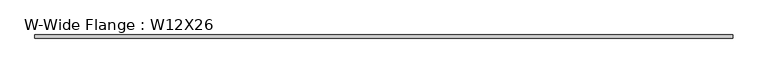
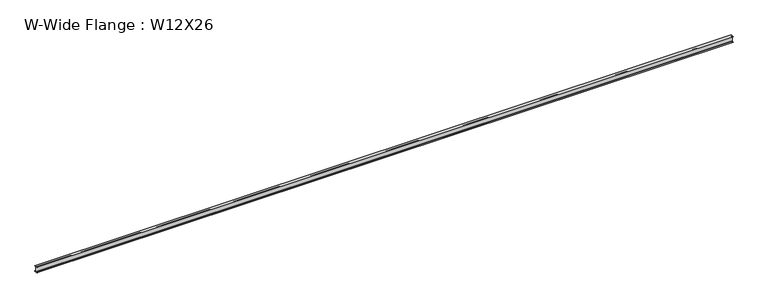
"""IFC4 building model written with IfcOpenShell, lengths in millimetres: beam geometry, W-Wide Flange : W12X26."""

from ifc_helpers import new_model, si_unit, point, frame, frame_2d, origin, place, context, project, spatial, polyline, circle_curve, trimmed, segment, composite_curve, outline, extrude, source, transform, mapped, element, save


def w_wide_flange_w12x26_694e4f9e(model_context):
    return source(origin(), model_context, "Body", "SweptSolid", [
        extrude(outline(composite_curve([segment(polyline([(82.4011719, -145.5539063), (82.4011719, -155.178125), (-82.4011719, -155.178125), (-82.4011719, -145.5539063), (-20.2902344, -145.5539063)]), True, "CONTINUOUS"), segment(trimmed(circle_curve(frame_2d((-20.2902344, -128.190625)), 17.3632812), [point((-20.2902344, -145.5539063))], [point((-2.9269531, -128.190625))], True, "CARTESIAN"), True, "CONTINUOUS"), segment(polyline([(-2.9269531, -128.190625), (-2.9269531, 128.190625)]), True, "CONTINUOUS"), segment(trimmed(circle_curve(frame_2d((-20.2902344, 128.190625)), 17.3632812), [point((-2.9269531, 128.190625))], [point((-20.2902344, 145.5539062))], True, "CARTESIAN"), True, "CONTINUOUS"), segment(polyline([(-20.2902344, 145.5539062), (-82.4011719, 145.5539062), (-82.4011719, 155.178125), (82.4011719, 155.178125), (82.4011719, 145.5539062), (20.2902344, 145.5539062)]), True, "CONTINUOUS"), segment(trimmed(circle_curve(frame_2d((20.2902344, 128.190625)), 17.3632812), [point((20.2902344, 145.5539062))], [point((2.9269531, 128.190625))], True, "CARTESIAN"), True, "CONTINUOUS"), segment(polyline([(2.9269531, 128.190625), (2.9269531, -128.190625)]), True, "CONTINUOUS"), segment(trimmed(circle_curve(frame_2d((20.2902344, -128.190625)), 17.3632812), [point((2.9269531, -128.190625))], [point((20.2902344, -145.5539063))], True, "CARTESIAN"), True, "CONTINUOUS"), segment(polyline([(20.2902344, -145.5539063), (82.4011719, -145.5539063)]), True, "CONTINUOUS")], self_intersect=False)), frame((-18165.7496628, 0.0, 0.0), z_axis=(1.0, 0.0, 0.0), x_axis=(0.0, 1.0, 0.0)), (0.0, 0.0, 1.0), 36331.4993256),
    ])


if __name__ == "__main__":
    model = new_model("IFC4")
    model_context = context("Model", 3, world=origin())
    ifc_project = project(units=[si_unit("LENGTHUNIT", "METRE", prefix="MILLI")], contexts=[model_context])
    site = spatial("IfcSite", under=ifc_project)
    building = spatial("IfcBuilding", under=site)
    placement = place(None, origin())
    w_wide_flange_w12x26_shape = w_wide_flange_w12x26_694e4f9e(model_context)
    element("IfcBeam", 1, ObjectType="W-Wide Flange : W12X26", at=placement, inside=building, context=model_context, shape_type="MappedRepresentation", body=[
        mapped(w_wide_flange_w12x26_shape, transform((0.0, 0.0, 0.0), x_axis=(1.0, 0.0, 0.0), y_axis=(0.0, 1.0, 0.0), z_axis=(0.0, 0.0, 1.0))),
    ])
    save(model, "model.ifc")

# Revit data of these elements
# Type "W-Wide Flange : W12X26"
#   Assembly Code = "B10"
#   W = 26
#   Length [instance default] = 5' - 0"
#   bf = 0' - 6 125/256"
#   d = 1' - 0 7/32"
#   k = 0' - 1 1/16"
#   k2 = 0' - 0 175/256"
#   tf = 0' - 0 97/256"
#   tw = 0' - 0 59/256"
#   A = 0.053125 SF
#   Structural Material [instance default] = none
# Element 1 (IfcBeam, "W-Wide Flange : W12X26")
#   Structural Material = Dark metal
#   Materials on its faces: "Dark metal"
# Materials
#   "Dark metal": class "Generic", colour RGB 44 29 29, transparency 0, Cost = 0
